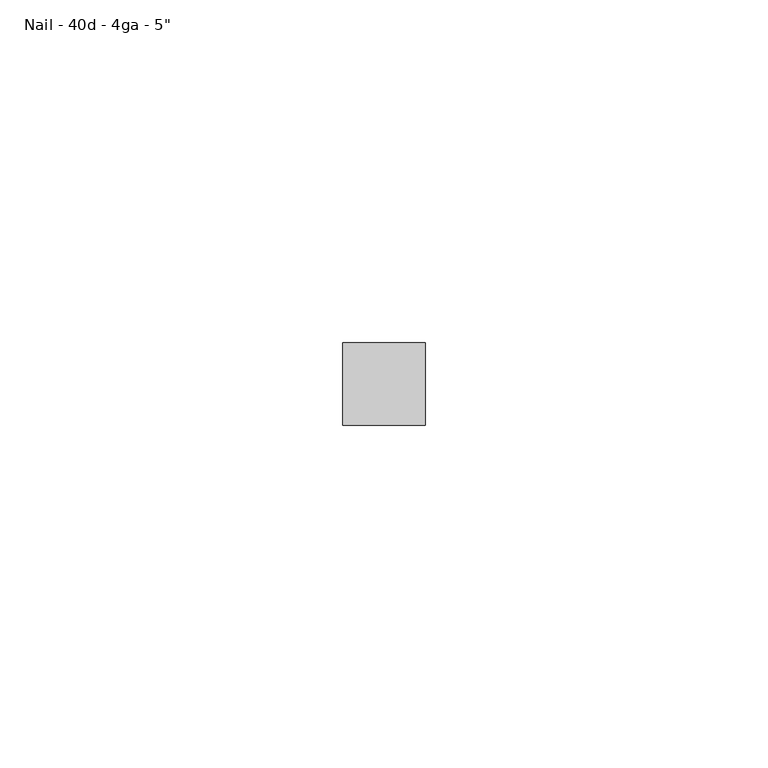
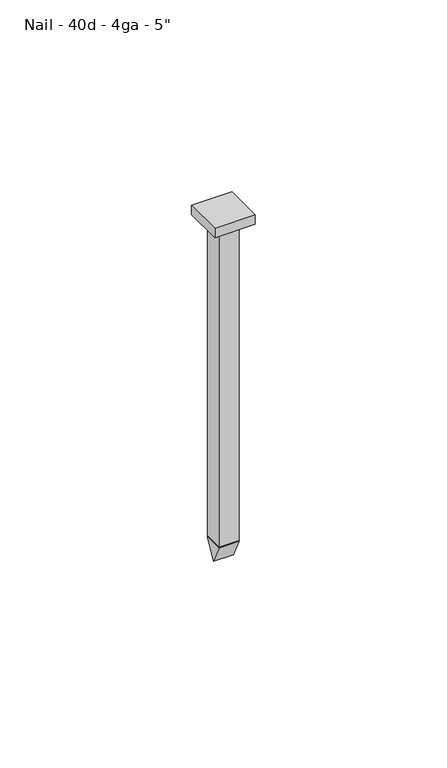
"""IFC4 building model written with IfcOpenShell, lengths in millimetres: fastener geometry."""

from ifc_helpers import new_model, si_unit, frame, origin, origin_with_axes, place, context, project, spatial, polyline, outline, extrude, source, transform, mapped, element, save


def fastener_ae3b06c6(model_context):
    return source(origin(), model_context, "Body", "SweptSolid", [
        extrude(outline(polyline([(0.0, -107.6452), (-3.0226, -101.6), (3.0226, -101.6), (0.0, -107.6452)])), frame((-3.0226, 0.0, 0.0), z_axis=(1.0, 0.0, 0.0), x_axis=(0.0, 1.0, 0.0)), (0.0, 0.0, 1.0), 6.0452),
        extrude(outline(polyline([(-6.0452, -6.0452), (-6.0452, 6.0452), (6.0452, 6.0452), (6.0452, -6.0452), (-6.0452, -6.0452)])), origin_with_axes(), (0.0, 0.0, 1.0), 3.0226),
        extrude(outline(polyline([(-3.0226, 3.0226), (3.0226, 3.0226), (3.0226, -3.0226), (-3.0226, -3.0226), (-3.0226, 3.0226)])), frame((0.0, 0.0, -101.6), z_axis=(0.0, 0.0, 1.0), x_axis=(1.0, 0.0, 0.0)), (0.0, 0.0, 1.0), 101.6),
    ])


if __name__ == "__main__":
    model = new_model("IFC4")
    model_context = context("Model", 3, world=origin())
    ifc_project = project(units=[si_unit("LENGTHUNIT", "METRE", prefix="MILLI")], contexts=[model_context])
    site = spatial("IfcSite", under=ifc_project)
    building = spatial("IfcBuilding", under=site)
    placement = place(None, origin())
    fastener_shape = fastener_ae3b06c6(model_context)
    element("IfcFastener", 1, ObjectType="060523 - W_P_C - Fastenings - Generic - SQUARE : Nail - 40d - 4ga - 5\"", at=placement, inside=building, context=model_context, shape_type="MappedRepresentation", body=[
        mapped(fastener_shape, transform((0.0, 0.0, 0.0), x_axis=(1.0, 0.0, 0.0), y_axis=(0.0, 1.0, 0.0), z_axis=(0.0, 0.0, 1.0))),
    ])
    save(model, "model.ifc")

# Revit data of these elements
# Type "060523 - W_P_C - Fastenings - Generic - SQUARE : Nail - 40d - 4ga - 5\""
#   Washer_Thickness = 0' - 0.00333"
#   Washer Radius = 0' - 0.129"
#   Washer Offset - Head = 0' - 0"
#   Washer Offset = 0' - 0"
#   Thickness_of_Substrate [instance default] = 0' - 1"
#   Side = 0' - 0 37/64"
#   Radius = 0' - 0.119"
#   Length [instance default] = 0' - 5"
#   Head Size = 0' - 1"
#   Head Radius = 0' - 0 1/2"
#   Head Height = 0' - 0.01"
#   Double Diameter = 0' - 0.476"
#   Diameter = 0' - 0.238"
#   Default Elevation = 4' - 0"
#   Washer_Nut_Visibility = no
#   Washer_Head_Visibility = no
#   Round_Head_Visibility = yes
#   Point Visibility = yes
#   Nut_Visibility = no
#   Hex_Head_Visiblilty = no
#   Washer Material = none
#   Bolt Material (Size) = AT SILL - FASTENER AT 24" O.C.
# Element 1 (IfcFastener, "060523 - W_P_C - Fastenings - Generic - SQUARE : Nail - 40d - 4ga - 5\"")
#   Length = 0' - 4"
# Materials
#   "AT SILL - FASTENER AT 24\" O.C.": class "Generic", colour RGB 120 120 120, transparency 0, Cost = 0
